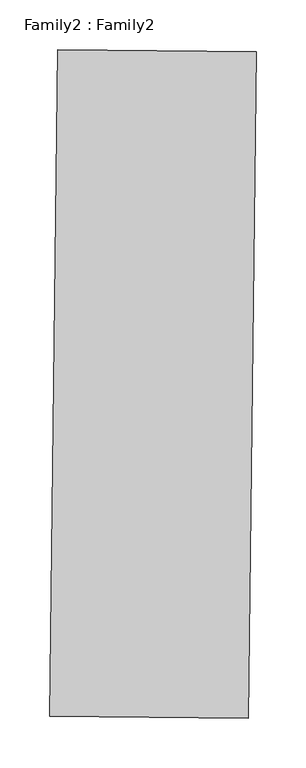
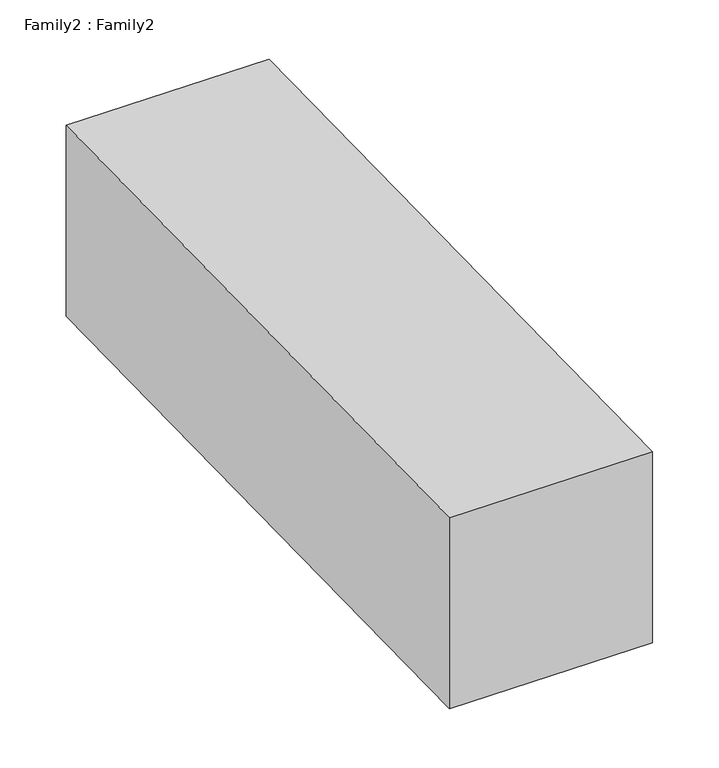
"""IFC4 building model written with IfcOpenShell, lengths in millimetres: proxy geometry, Family2 : Family2."""

from ifc_helpers import new_model, si_unit, origin, place, context, project, spatial, faceted_brep, source, transform, mapped, element, save


def family2_family2_5d0bf995(model_context):
    return source(origin(), model_context, "Body", "Brep", [
        faceted_brep([(-3947.3850716, -6409.2935888, 1.0945136), (-3947.3850716, -6409.2935888, 201.0945136), (-3939.4577229, -5738.3065338, 202.060409), (-3939.4577229, -5738.3065338, 2.060409), (-3747.3938816, -6411.1708015, 201.0945136), (-3739.4665329, -5740.1837465, 202.060409), (-3747.3938816, -6411.1708015, 1.0945136), (-3739.4665329, -5740.1837465, 2.060409)], [[[0, 1, 2, 3]], [[1, 4, 5, 2]], [[4, 6, 7, 5]], [[6, 0, 3, 7]], [[3, 2, 5, 7]], [[0, 6, 4, 1]]]),
    ])


if __name__ == "__main__":
    model = new_model("IFC4")
    model_context = context("Model", 3, world=origin())
    ifc_project = project(units=[si_unit("LENGTHUNIT", "METRE", prefix="MILLI")], contexts=[model_context])
    site = spatial("IfcSite", under=ifc_project)
    building = spatial("IfcBuilding", under=site)
    placement = place(None, origin())
    family2_family2_shape = family2_family2_5d0bf995(model_context)
    element("IfcBuildingElementProxy", 1, Name="Family2 : Family2", ObjectType="Family2 : Family2", at=placement, inside=building, context=model_context, shape_type="MappedRepresentation", body=[
        mapped(family2_family2_shape, transform((0.0, 0.0, 0.0), x_axis=(1.0, 0.0, 0.0), y_axis=(0.0, 1.0, 0.0), z_axis=(0.0, 0.0, 1.0))),
    ])
    save(model, "model.ifc")

# Revit data of these elements
# Type "Family2 : Family2"
#   Default Elevation = 0
